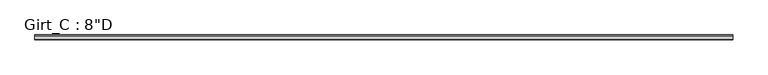
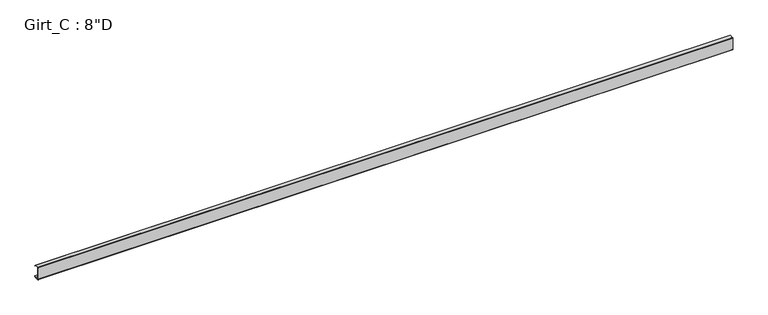
"""IFC4 building model written with IfcOpenShell, lengths in millimetres: beam geometry."""

from ifc_helpers import new_model, si_unit, point, frame, frame_2d, origin, place, context, project, spatial, polyline, circle_curve, trimmed, segment, composite_curve, outline, extrude, source, transform, mapped, element, save


def beam_08470fd9(model_context):
    return source(origin(), model_context, "Body", "SweptSolid", [
        extrude(outline(composite_curve([segment(polyline([(63.5, 101.6), (75.745104, 87.0068534), (73.6169367, 85.221109), (62.204539, 98.821875), (3.3005807, 98.821875)]), True, "CONTINUOUS"), segment(trimmed(circle_curve(frame_2d((3.3741066, 96.8381931)), 1.9850441), [point((3.3005807, 98.821875))], [point((1.3890625, 96.8381931))], True, "CARTESIAN"), True, "CONTINUOUS"), segment(polyline([(1.3890625, 96.8381931), (1.3890625, -96.8389339)]), True, "CONTINUOUS"), segment(trimmed(circle_curve(frame_2d((3.3748024, -96.8389339)), 1.9857399), [point((1.3890625, -96.8389339))], [point((3.2694106, -98.821875))], True, "CARTESIAN"), True, "CONTINUOUS"), segment(polyline([(3.2694106, -98.821875), (62.204539, -98.821875), (73.6169367, -85.221109), (75.745104, -87.0068534), (63.5, -101.6), (3.3734375, -101.6)]), True, "CONTINUOUS"), segment(trimmed(circle_curve(frame_2d((3.3734375, -96.8375)), 4.7625), [point((3.3734375, -101.6))], [point((-1.3890625, -96.8375))], False, "CARTESIAN"), True, "CONTINUOUS"), segment(polyline([(-1.3890625, -96.8375), (-1.3890625, 96.8375)]), True, "CONTINUOUS"), segment(trimmed(circle_curve(frame_2d((3.3734375, 96.8375)), 4.7625), [point((-1.3890625, 96.8375))], [point((3.3734375, 101.6))], False, "CARTESIAN"), True, "CONTINUOUS"), segment(polyline([(3.3734375, 101.6), (63.5, 101.6)]), True, "CONTINUOUS")], self_intersect=False)), frame((-5514.975, 0.0, 0.0), z_axis=(1.0, 0.0, 0.0), x_axis=(0.0, 1.0, 0.0)), (0.0, 0.0, 1.0), 10963.275),
    ])


if __name__ == "__main__":
    model = new_model("IFC4")
    model_context = context("Model", 3, world=origin())
    ifc_project = project(units=[si_unit("LENGTHUNIT", "METRE", prefix="MILLI")], contexts=[model_context])
    site = spatial("IfcSite", under=ifc_project)
    building = spatial("IfcBuilding", under=site)
    placement = place(None, origin())
    beam_shape = beam_08470fd9(model_context)
    element("IfcBeam", 1, ObjectType="Girt_C : 8\"D", at=placement, inside=building, context=model_context, shape_type="MappedRepresentation", body=[
        mapped(beam_shape, transform((0.0, 0.0, 0.0), x_axis=(1.0, 0.0, 0.0), y_axis=(0.0, 1.0, 0.0), z_axis=(0.0, 0.0, 1.0))),
    ])
    save(model, "model.ifc")

# Revit data of these elements
# Type "Girt_C : 8\"D"
#   Web_Thickness = 0' - 0 7/64"
#   Length [instance default] = 10' - 0"
#   Leg_1 = 0' - 2 1/2"
#   Height = 0' - 8"
#   Structural Material [instance default] = none
